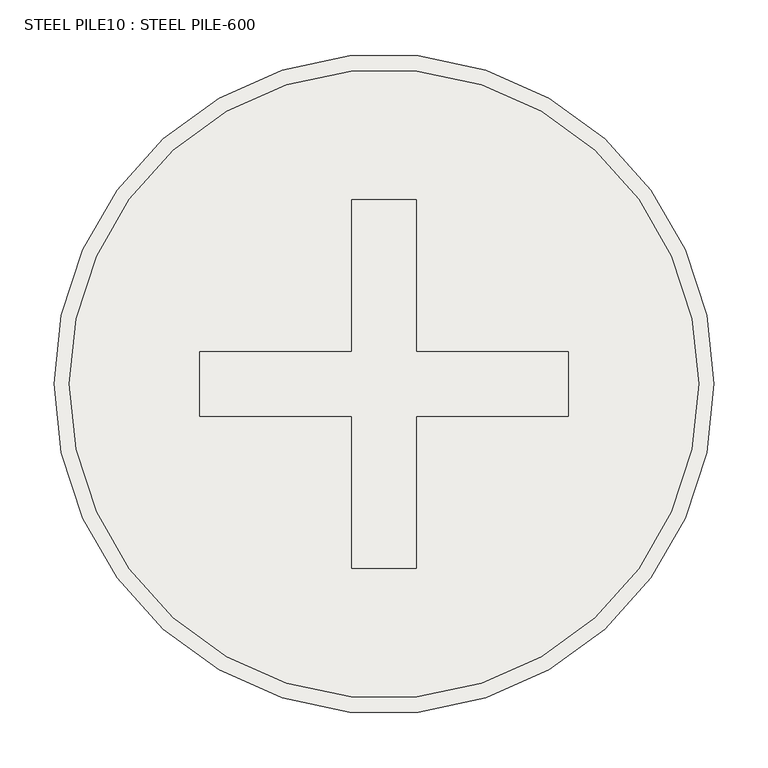
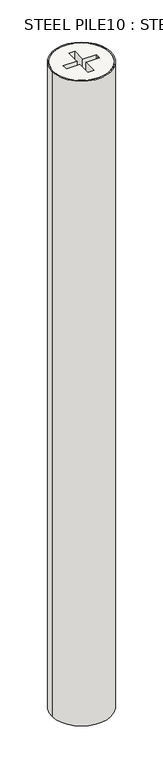
"""IFC4 building model written with IfcOpenShell, lengths in millimetres: slab geometry, STEEL PILE10 : STEEL PILE-600."""

from ifc_helpers import new_model, si_unit, point, frame, frame_2d, origin, place, context, project, spatial, circle_curve, trimmed, segment, composite_curve, outline, extrude, source, transform, mapped, element, save
from ifc_brep_helpers import plane_surface, cylinder_surface, advanced_brep


def steel_pile10_steel_pile_600_aa0c33d1(model_context):
    return source(origin(), model_context, "Body", "SolidModel", [
        advanced_brep(
        [(5709.5, 22499.5208589, 150.0), (6290.5, 22499.5208589, 150.0), (5970.0, 22469.5208589, 150.0), (5830.0, 22469.5208589, 150.0), (5830.0, 22499.5208589, 150.0), (5830.0, 22529.5208589, 150.0), (5970.0, 22529.5208589, 150.0), (5970.0, 22669.5208589, 150.0), (6030.0, 22669.5208589, 150.0), (6030.0, 22529.5208589, 150.0), (6170.0, 22529.5208589, 150.0), (6170.0, 22499.5208589, 150.0), (6170.0, 22469.5208589, 150.0), (6030.0, 22469.5208589, 150.0), (6030.0, 22329.5208589, 150.0), (5970.0, 22329.5208589, 150.0), (5709.5, 22499.5208589, -1850.0), (6290.5, 22499.5208589, -1850.0), (5830.0, 22469.5208589, -160.0), (5970.0, 22469.5208589, -160.0), (5970.0, 22329.5208589, -160.0), (6030.0, 22329.5208589, -160.0), (6030.0, 22469.5208589, -160.0), (6170.0, 22469.5208589, -160.0), (6170.0, 22499.5208589, -160.0), (6170.0, 22529.5208589, -160.0), (6030.0, 22529.5208589, -160.0), (6030.0, 22669.5208589, -160.0), (5970.0, 22669.5208589, -160.0), (5970.0, 22529.5208589, -160.0), (5830.0, 22529.5208589, -160.0), (5830.0, 22499.5208589, -160.0)],
        [
            (0, 1, circle_curve(frame((6000.0, 22499.5208589, 150.0), z_axis=(0.0, 0.0, 1.0), x_axis=(1.0, 0.0, 0.0)), 290.5)),
            (1, 0, circle_curve(frame((6000.0, 22499.5208589, 150.0), z_axis=(0.0, 0.0, 1.0), x_axis=(1.0, 0.0, 0.0)), 290.5)),
            (2, 3),
            (3, 4),
            (4, 5),
            (5, 6),
            (6, 7),
            (7, 8),
            (8, 9),
            (9, 10),
            (10, 11),
            (11, 12),
            (12, 13),
            (13, 14),
            (14, 15),
            (15, 2),
            (16, 17, circle_curve(frame((6000.0, 22499.5208589, -1850.0), z_axis=(0.0, 0.0, -1.0), x_axis=(1.0, 0.0, 0.0)), 290.5)),
            (17, 16, circle_curve(frame((6000.0, 22499.5208589, -1850.0), z_axis=(0.0, 0.0, -1.0), x_axis=(1.0, 0.0, 0.0)), 290.5)),
            (0, 16),
            (17, 1),
            (18, 19),
            (19, 20),
            (20, 21),
            (21, 22),
            (22, 23),
            (23, 24),
            (24, 25),
            (25, 26),
            (26, 27),
            (27, 28),
            (28, 29),
            (29, 30),
            (30, 31),
            (31, 18),
            (18, 3),
            (2, 19),
            (15, 20),
            (14, 21),
            (13, 22),
            (12, 23),
            (11, 24),
            (10, 25),
            (9, 26),
            (8, 27),
            (7, 28),
            (6, 29),
            (5, 30),
            (4, 31),
        ],
        [
            plane_surface(frame((6290.5, 22499.5208589, 150.0), z_axis=(0.0, 0.0, 1.0), x_axis=(0.0, 1.0, 0.0))),
            plane_surface(frame((6290.5, 22499.5208589, -1850.0), z_axis=(0.0, 0.0, -1.0), x_axis=(0.0, -1.0, 0.0))),
            cylinder_surface(frame((6000.0, 22499.5208589, -1850.0), z_axis=(0.0, 0.0, 1.0), x_axis=(1.0, 0.0, 0.0)), 290.5),
            plane_surface(frame((5830.0, 22469.5208589, -160.0), z_axis=(0.0, 0.0, 1.0), x_axis=(-1.0, 0.0, 0.0))),
            plane_surface(frame((5830.0, 22469.5208589, 160.0), z_axis=(0.0, 1.0, 0.0), x_axis=(0.0, 0.0, -1.0))),
            plane_surface(frame((5970.0, 22469.5208589, 160.0), z_axis=(1.0, 0.0, 0.0), x_axis=(0.0, 0.0, -1.0))),
            plane_surface(frame((5970.0, 22329.5208589, 160.0), z_axis=(0.0, 1.0, 0.0), x_axis=(0.0, 0.0, -1.0))),
            plane_surface(frame((6030.0, 22329.5208589, 160.0), z_axis=(-1.0, 0.0, 0.0), x_axis=(0.0, 0.0, -1.0))),
            plane_surface(frame((6030.0, 22469.5208589, 160.0), z_axis=(0.0, 1.0, 0.0), x_axis=(0.0, 0.0, -1.0))),
            plane_surface(frame((6170.0, 22469.5208589, 160.0), z_axis=(-1.0, 0.0, 0.0), x_axis=(0.0, 0.0, -1.0))),
            plane_surface(frame((6170.0, 22499.5208589, 160.0), z_axis=(-1.0, 0.0, 0.0), x_axis=(0.0, 0.0, -1.0))),
            plane_surface(frame((6170.0, 22529.5208589, 160.0), z_axis=(0.0, -1.0, 0.0), x_axis=(0.0, 0.0, -1.0))),
            plane_surface(frame((6030.0, 22529.5208589, 160.0), z_axis=(-1.0, 0.0, 0.0), x_axis=(0.0, 0.0, -1.0))),
            plane_surface(frame((6030.0, 22669.5208589, 160.0), z_axis=(0.0, -1.0, 0.0), x_axis=(0.0, 0.0, -1.0))),
            plane_surface(frame((5970.0, 22669.5208589, 160.0), z_axis=(1.0, 0.0, 0.0), x_axis=(0.0, 0.0, -1.0))),
            plane_surface(frame((5970.0, 22529.5208589, 160.0), z_axis=(0.0, -1.0, 0.0), x_axis=(0.0, 0.0, -1.0))),
            plane_surface(frame((5830.0, 22529.5208589, 160.0), z_axis=(1.0, 0.0, 0.0), x_axis=(0.0, 0.0, -1.0))),
            plane_surface(frame((5830.0, 22499.5208589, 160.0), z_axis=(1.0, 0.0, 0.0), x_axis=(0.0, 0.0, -1.0))),
        ],
        [
            (0, [[1, 2], [3, 4, 5, 6, 7, 8, 9, 10, 11, 12, 13, 14, 15, 16]]),
            (1, [[17, 18]]),
            (2, [[-1, 19, -18, 20]]),
            (2, [[-2, -20, -17, -19]]),
            (3, [[21, 22, 23, 24, 25, 26, 27, 28, 29, 30, 31, 32, 33, 34]]),
            (4, [[-21, 35, -3, 36]]),
            (5, [[-22, -36, -16, 37]]),
            (6, [[-23, -37, -15, 38]]),
            (7, [[-24, -38, -14, 39]]),
            (8, [[-25, -39, -13, 40]]),
            (9, [[-26, -40, -12, 41]]),
            (10, [[-27, -41, -11, 42]]),
            (11, [[-28, -42, -10, 43]]),
            (12, [[-29, -43, -9, 44]]),
            (13, [[-30, -44, -8, 45]]),
            (14, [[-31, -45, -7, 46]]),
            (15, [[-32, -46, -6, 47]]),
            (16, [[-33, -47, -5, 48]]),
            (17, [[-34, -48, -4, -35]]),
        ],
    ),
        extrude(outline(composite_curve([segment(trimmed(circle_curve(frame_2d((6000.0, 22499.5208589)), 304.5), [point((5695.5, 22499.5208589))], [point((6304.5, 22499.5208589))], False, "CARTESIAN"), True, "CONTINUOUS"), segment(trimmed(circle_curve(frame_2d((6000.0, 22499.5208589)), 304.5), [point((6304.5, 22499.5208589))], [point((5695.5, 22499.5208589))], False, "CARTESIAN"), True, "CONTINUOUS")], self_intersect=False), holes=[composite_curve([segment(trimmed(circle_curve(frame_2d((6000.0, 22499.5208589)), 290.5), [point((5709.5, 22499.5208589))], [point((6290.5, 22499.5208589))], True, "CARTESIAN"), True, "CONTINUOUS"), segment(trimmed(circle_curve(frame_2d((6000.0, 22499.5208589)), 290.5), [point((6290.5, 22499.5208589))], [point((5709.5, 22499.5208589))], True, "CARTESIAN"), True, "CONTINUOUS")], self_intersect=False)]), frame((0.0, 0.0, -6850.0), z_axis=(0.0, 0.0, 1.0), x_axis=(1.0, 0.0, 0.0)), (0.0, 0.0, 1.0), 7000.0),
    ])


if __name__ == "__main__":
    model = new_model("IFC4")
    model_context = context("Model", 3, world=origin())
    ifc_project = project(units=[si_unit("LENGTHUNIT", "METRE", prefix="MILLI")], contexts=[model_context])
    site = spatial("IfcSite", under=ifc_project)
    building = spatial("IfcBuilding", under=site)
    placement = place(None, origin())
    steel_pile10_steel_pile_600_shape = steel_pile10_steel_pile_600_aa0c33d1(model_context)
    element("IfcSlab", 1, ObjectType="STEEL PILE10 : STEEL PILE-600", at=placement, inside=building, context=model_context, shape_type="MappedRepresentation", body=[
        mapped(steel_pile10_steel_pile_600_shape, transform((0.0, 0.0, 0.0), x_axis=(1.0, 0.0, 0.0), y_axis=(0.0, 1.0, 0.0), z_axis=(0.0, 0.0, 1.0))),
    ])
    save(model, "model.ifc")
